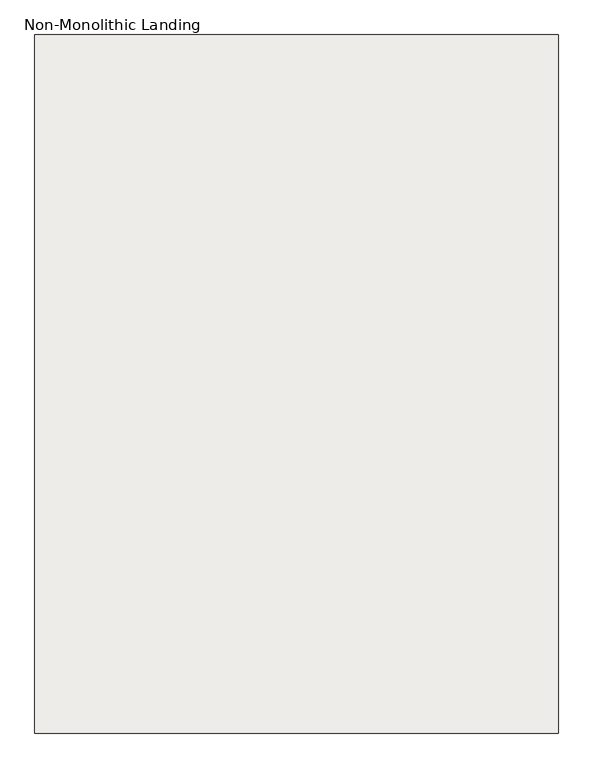
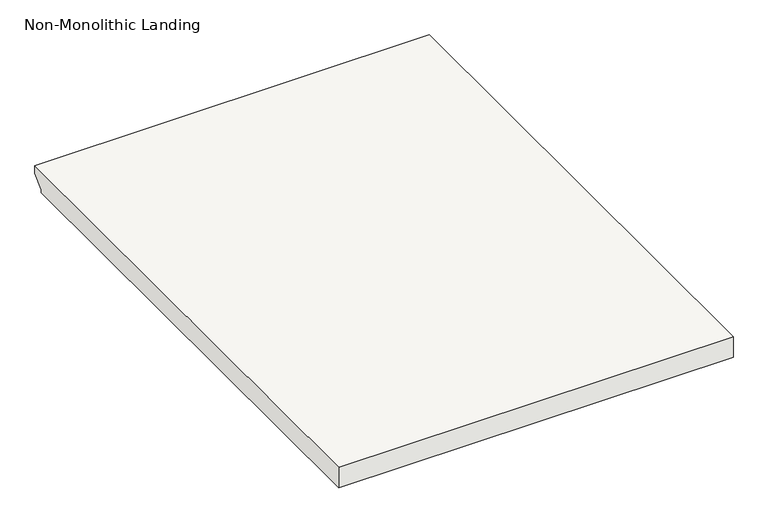
"""IFC4 building model written with IfcOpenShell, lengths in millimetres: slab geometry, Non-Monolithic Landing."""

from ifc_helpers import new_model, si_unit, frame, origin, place, context, project, spatial, polyline, outline, extrude, source, transform, mapped, element, save


def non_monolithic_landing_25f7bf71(model_context):
    return source(origin(), model_context, "Body", "SweptSolid", [
        extrude(outline(polyline([(13666.8483822, 3048.0), (14886.0483822, 3048.0), (14886.0483822, 3028.95), (14860.6483822, 3003.55), (14860.6483822, 2997.2), (13666.8483822, 2997.2), (13666.8483822, 3048.0)])), frame((16081.5123343, 0.0, 0.0), z_axis=(1.0, 0.0, 0.0), x_axis=(0.0, 1.0, 0.0)), (0.0, 0.0, 1.0), 914.4),
    ])


if __name__ == "__main__":
    model = new_model("IFC4")
    model_context = context("Model", 3, world=origin())
    ifc_project = project(units=[si_unit("LENGTHUNIT", "METRE", prefix="MILLI")], contexts=[model_context])
    site = spatial("IfcSite", under=ifc_project)
    building = spatial("IfcBuilding", under=site)
    placement = place(None, origin())
    non_monolithic_landing_shape = non_monolithic_landing_25f7bf71(model_context)
    element("IfcSlab", 1, ObjectType="Non-Monolithic Landing", at=placement, inside=building, context=model_context, shape_type="MappedRepresentation", body=[
        mapped(non_monolithic_landing_shape, transform((0.0, 0.0, 0.0), x_axis=(1.0, 0.0, 0.0), y_axis=(0.0, 1.0, 0.0), z_axis=(0.0, 0.0, 1.0))),
    ])
    save(model, "model.ifc")

# Revit data of these elements
# Element 1 (IfcSlab, "Non-Monolithic Landing")
#   Materials on its faces: "Oak Flooring"
# Materials
#   "Oak Flooring": class "Wood", colour RGB 216 169 114, transparency 0, Description = "Quercus Rubra", Cost = 0
